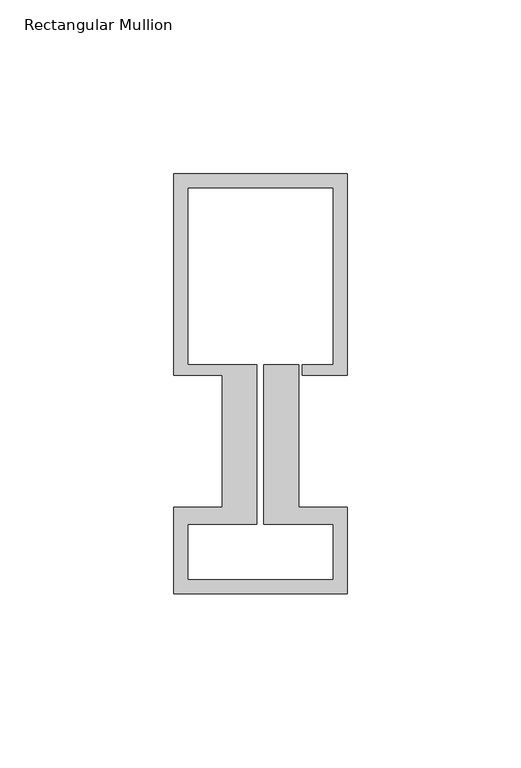
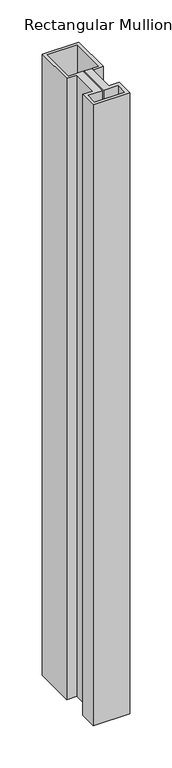
"""IFC4 building model written with IfcOpenShell, lengths in millimetres: member geometry, Rectangular Mullion : Schueco_FWS-50-SI_Tran_CovCap-20mm_Tran-55mm."""

from ifc_helpers import new_model, si_unit, frame, origin, place, context, project, spatial, polyline, outline, extrude, source, transform, mapped, element, save


def rectangular_mullion_7e76487e(model_context):
    return source(origin(), model_context, "Body", "SweptSolid", [
        extrude(outline(polyline([(-50.0, 96.0), (0.0, 96.0), (0.0, 38.0), (-13.0, 38.0), (-13.0, 41.0), (-4.0, 41.0), (-4.0, 92.0), (-46.0, 92.0), (-46.0, 41.0), (-26.0, 41.0), (-26.0, -5.0), (-46.0, -5.0), (-46.0, -21.0), (-4.0, -21.0), (-4.0, -5.0), (-24.0, -5.0), (-24.0, 41.0), (-14.0, 41.0), (-14.0, -0.1), (0.0, -0.1), (0.0, -25.0), (-50.0, -25.0), (-50.0, -0.1), (-36.0, -0.1), (-36.0, 38.0), (-50.0, 38.0), (-50.0, 96.0)])), frame((0.0, 0.0, -900.0), z_axis=(0.0, 0.0, 1.0), x_axis=(1.0, 0.0, 0.0)), (0.0, 0.0, 1.0), 900.0),
    ])


if __name__ == "__main__":
    model = new_model("IFC4")
    model_context = context("Model", 3, world=origin())
    ifc_project = project(units=[si_unit("LENGTHUNIT", "METRE", prefix="MILLI")], contexts=[model_context])
    site = spatial("IfcSite", under=ifc_project)
    building = spatial("IfcBuilding", under=site)
    placement = place(None, origin())
    rectangular_mullion_shape = rectangular_mullion_7e76487e(model_context)
    element("IfcMember", 1, ObjectType="Rectangular Mullion : Schueco_FWS-50-SI_Tran_CovCap-20mm_Tran-55mm", at=placement, inside=building, context=model_context, shape_type="MappedRepresentation", body=[
        mapped(rectangular_mullion_shape, transform((0.0, 0.0, 0.0), x_axis=(1.0, 0.0, 0.0), y_axis=(0.0, 1.0, 0.0), z_axis=(0.0, 0.0, 1.0))),
    ])
    save(model, "model.ifc")

# Revit data of these elements
# Type "Rectangular Mullion : Schueco_FWS-50-SI_Tran_CovCap-20mm_Tran-55mm"
#   Model = "FWS 50.SI"
#   Manufacturer = "Schueco International KG"
#   Type Comments = "Transom"
#   Schueco thermal insulation standard = "Suitable for passive houses"
#   Burglar resistance = "RC 3"
#   Thermal insulation = "to 0.70 W/(m²K)"
#   built-in parameter 1007322 = 0.396982 (stored number, unit not read)
#   built-in parameter 1007321 = 0.0360892 (stored number, unit not read)
#   built-in parameter 1007320 = 0.0360892 (stored number, unit not read)
# Element 1 (IfcMember, "Rectangular Mullion : Schueco_FWS-50-SI_Tran_CovCap-20mm_Tran-55mm")
#   Materials on its faces: "Alu"
# Materials
#   "Alu": class "Glas", colour RGB 140 140 140, transparency 0
